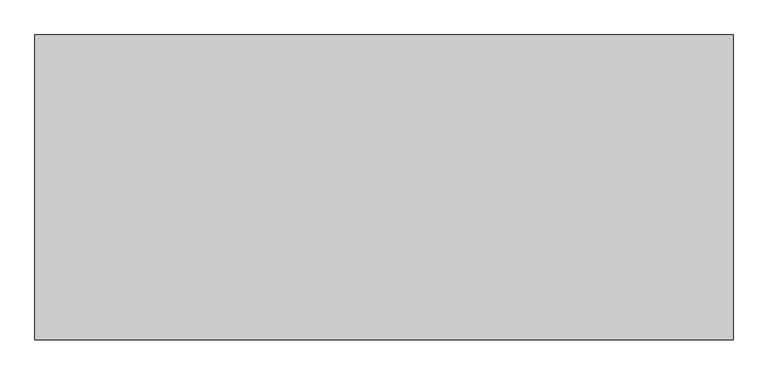
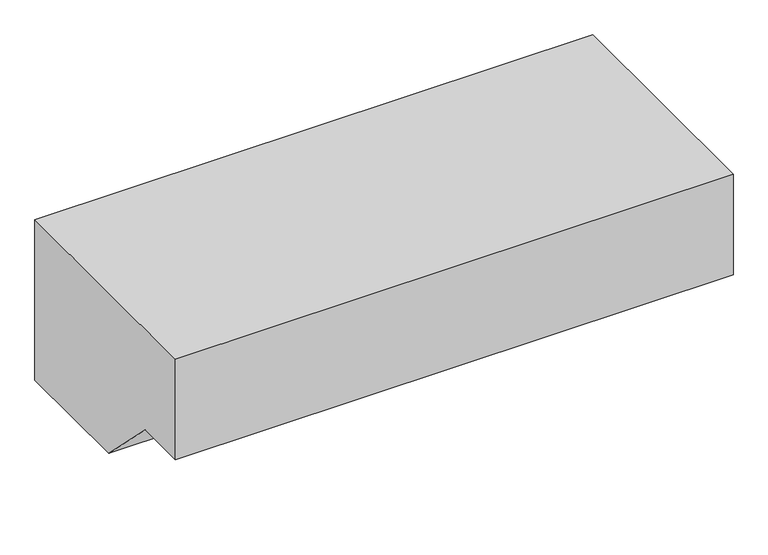
"""IFC4 building model written with IfcOpenShell, lengths in millimetres: proxy geometry, Slab001 1434 : Slab001 1434."""

from ifc_helpers import new_model, si_unit, frame, origin, place, context, project, spatial, polyline, outline, extrude, source, transform, mapped, element, save


def generic_models_17c20b3a(model_context):
    return source(origin(), model_context, "Body", "SweptSolid", [
        extrude(outline(polyline([(9730.3375834, 36531.296), (9730.3375834, 35921.696), (9273.1375834, 35921.696), (9044.5375834, 36150.296), (8857.5938813, 36150.296), (8857.5938813, 36531.296), (9730.3375834, 36531.296)])), frame((3694.2883192, 0.0, 0.0), z_axis=(1.0, 0.0, 0.0), x_axis=(0.0, 1.0, 0.0)), (0.0, 0.0, 1.0), 2000.0),
    ])


if __name__ == "__main__":
    model = new_model("IFC4")
    model_context = context("Model", 3, world=origin())
    ifc_project = project(units=[si_unit("LENGTHUNIT", "METRE", prefix="MILLI")], contexts=[model_context])
    site = spatial("IfcSite", under=ifc_project)
    building = spatial("IfcBuilding", under=site)
    placement = place(None, origin())
    generic_models_shape = generic_models_17c20b3a(model_context)
    element("IfcBuildingElementProxy", 1, Name="Slab001 1434 : Slab001 1434", ObjectType="Slab001 1434 : Slab001 1434", at=placement, inside=building, context=model_context, shape_type="MappedRepresentation", body=[
        mapped(generic_models_shape, transform((0.0, 0.0, 0.0), x_axis=(1.0, 0.0, 0.0), y_axis=(0.0, 1.0, 0.0), z_axis=(0.0, 0.0, 1.0))),
    ])
    save(model, "model.ifc")

# Revit data of these elements
# Type "Slab001 1434 : Slab001 1434"
#   NameOverride = "Slab001"
# Element 1 (IfcBuildingElementProxy, "Slab001 1434 : Slab001 1434")
#   Materials on its faces: "CONCRETE SLAB W/ GRADE BEAM (SEE STRUCT DWGS)"
# Materials
#   "CONCRETE SLAB W/ GRADE BEAM (SEE STRUCT DWGS)": class "Unassigned", colour RGB 128 128 128, transparency 0, Cost = 0
